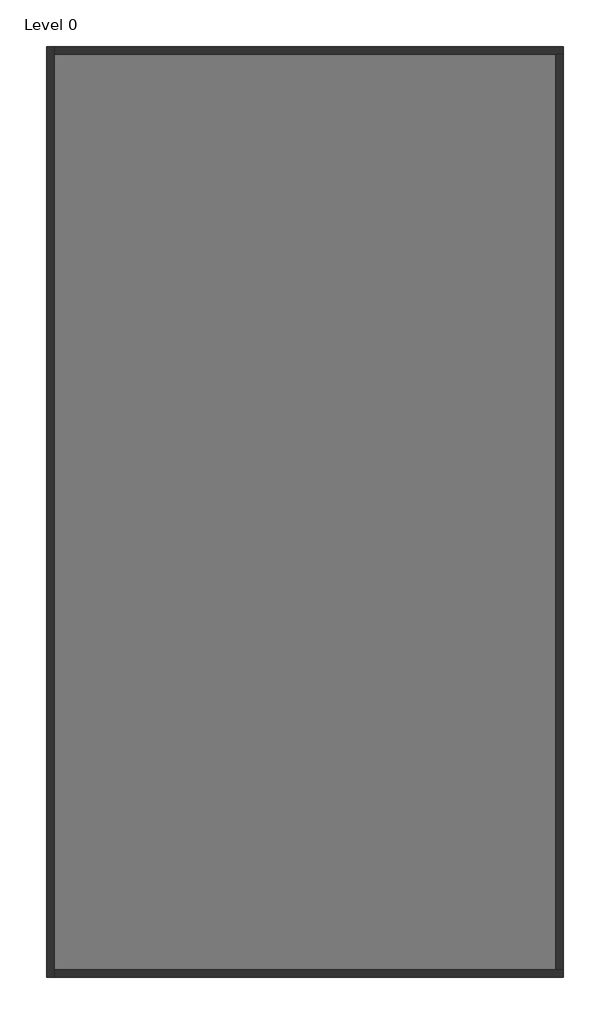
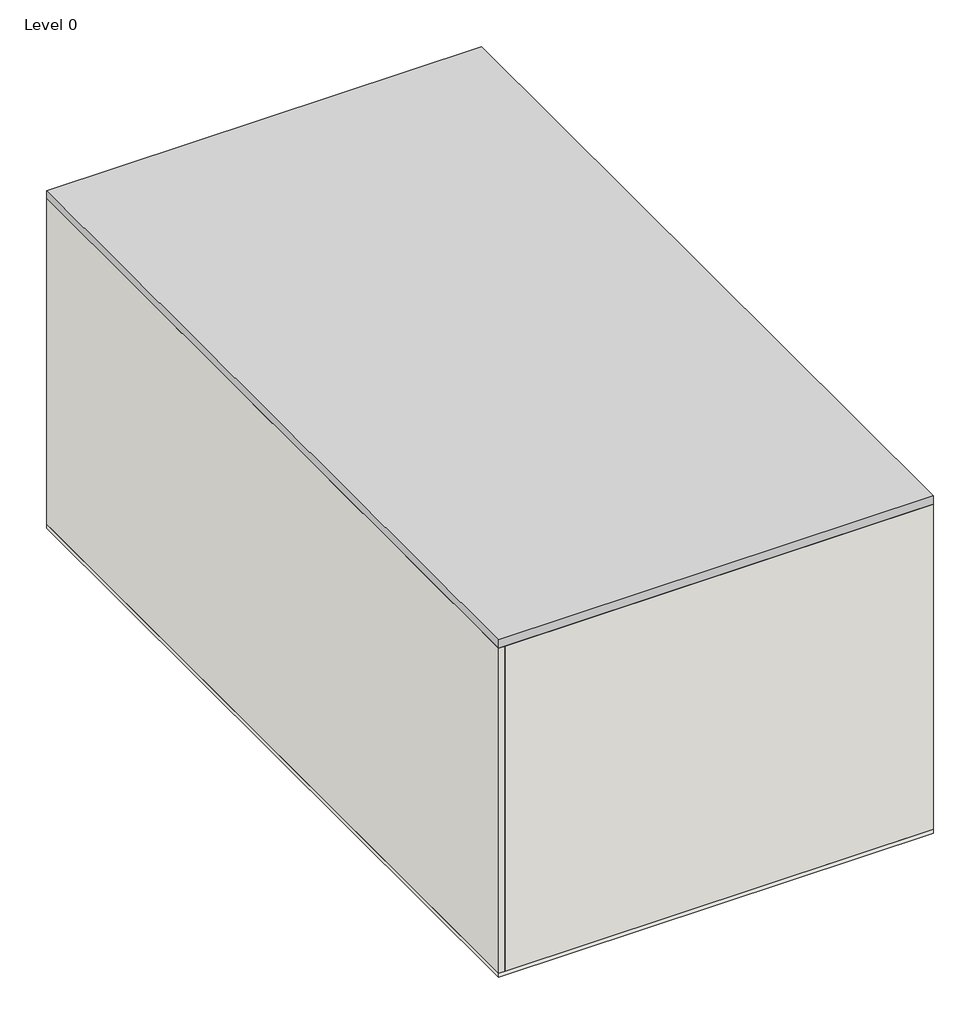
# One storey: 4 walls, 1 proxy, 1 slab.
"""IFC4 building model written with IfcOpenShell, lengths in millimetres."""

from ifc_helpers import new_model, si_unit, frame, origin, origin_with_axes, place, context, project, spatial, polyline, outline, extrude, faceted_brep, element, save

model = new_model("IFC4")

# Units and contexts
model_context = context("Model", 3, world=origin())
ifc_project = project(units=[si_unit("LENGTHUNIT", "METRE", prefix="MILLI")], contexts=[model_context])

# Site, building, storey
site = spatial("IfcSite", under=ifc_project)
building = spatial("IfcBuilding", under=site)
storey = spatial("IfcBuildingStorey", under=building, Name="Level 0", Elevation=100.0)

# Proxy
placement = place(None, origin())
element("IfcBuildingElementProxy", 1, Name="LowUrbanDensityBuilding : LowUrbanDensityBuilding", ObjectType="LowUrbanDensityBuilding : LowUrbanDensityBuilding", at=placement, inside=storey, context=model_context, shape_type="SweptSolid", body=[
    extrude(outline(polyline([(7325.2659446, 3676.2074539), (7325.2659446, -14323.7925461), (-2674.7340554, -14323.7925461), (-2674.7340554, 3676.2074539), (7325.2659446, 3676.2074539)])), origin_with_axes(), (0.0, 0.0, 1.0), 8200.0),
])

# Slab
element("IfcSlab", 2, ObjectType="Floor-Concrete_100Con", at=placement, inside=storey, context=model_context, shape_type="SweptSolid", body=[
    extrude(outline(polyline([(7325.2659446, 3676.2074539), (7325.2659446, -14323.7925461), (-2674.7340554, -14323.7925461), (-2674.7340554, 3676.2074539), (7325.2659446, 3676.2074539)])), origin_with_axes(), (0.0, 0.0, 1.0), 100.0),
])

# Walls
element("IfcWall", 3, ObjectType="Wall-Ext_25Rdr-100Blk-19P", at=placement, inside=storey, context=model_context, shape_type="Brep", body=[
    faceted_brep([(-2674.7340554, 3676.2074539, 100.0), (-2674.7340554, -14323.7925461, 100.0), (-2674.7340554, -14323.7925461, 8000.0), (-2674.7340554, 3676.2074539, 8000.0), (-2530.4340554, 3676.2074539, 100.0), (-2530.4340554, 3676.2074539, 8000.0), (-2530.4340554, 3531.9074539, 8000.0), (-2530.4340554, -14179.4925461, 8000.0), (-2530.4340554, -14323.7925461, 8000.0), (-2530.4340554, -14323.7925461, 100.0), (-2530.4340554, -14179.4925461, 100.0), (-2530.4340554, 3531.9074539, 100.0)], [[[0, 1, 2, 3]], [[4, 5, 6, 7, 8, 9, 10, 11]], [[1, 0, 4, 11, 10, 9]], [[3, 2, 8, 7, 6, 5]], [[2, 1, 9, 8]], [[0, 3, 5, 4]]]),
])
element("IfcWall", 4, ObjectType="Wall-Ext_25Rdr-100Blk-19P", at=placement, inside=storey, context=model_context, shape_type="Brep", body=[
    faceted_brep([(-2530.4340554, -14323.7925461, 100.0), (7325.2659446, -14323.7925461, 100.0), (7325.2659446, -14323.7925461, 8000.0), (-2530.4340554, -14323.7925461, 8000.0), (-2530.4340554, -14179.4925461, 100.0), (-2530.4340554, -14179.4925461, 8000.0), (7180.9659446, -14179.4925461, 8000.0), (7325.2659446, -14179.4925461, 8000.0), (7325.2659446, -14179.4925461, 100.0), (7180.9659446, -14179.4925461, 100.0)], [[[0, 1, 2, 3]], [[4, 5, 6, 7, 8, 9]], [[1, 0, 4, 9, 8]], [[3, 2, 7, 6, 5]], [[0, 3, 5, 4]], [[2, 1, 8, 7]]]),
])
element("IfcWall", 5, ObjectType="Wall-Ext_25Rdr-100Blk-19P", at=placement, inside=storey, context=model_context, shape_type="Brep", body=[
    faceted_brep([(7325.2659446, 3676.2074539, 100.0), (-2530.4340554, 3676.2074539, 100.0), (-2530.4340554, 3676.2074539, 8000.0), (7325.2659446, 3676.2074539, 8000.0), (7325.2659446, 3531.9074539, 100.0), (7325.2659446, 3531.9074539, 8000.0), (7180.9659446, 3531.9074539, 8000.0), (-2530.4340554, 3531.9074539, 8000.0), (-2530.4340554, 3531.9074539, 100.0), (7180.9659446, 3531.9074539, 100.0)], [[[0, 1, 2, 3]], [[4, 5, 6, 7, 8, 9]], [[1, 0, 4, 9, 8]], [[3, 2, 7, 6, 5]], [[2, 1, 8, 7]], [[0, 3, 5, 4]]]),
])
element("IfcWall", 6, ObjectType="Wall-Ext_25Rdr-100Blk-19P", at=placement, inside=storey, context=model_context, shape_type="SweptSolid", body=[
    extrude(outline(polyline([(7325.2659446, 3531.9074539), (7325.2659446, -14179.4925461), (7180.9659446, -14179.4925461), (7180.9659446, 3531.9074539), (7325.2659446, 3531.9074539)])), frame((0.0, 0.0, 100.0), z_axis=(0.0, 0.0, 1.0), x_axis=(1.0, 0.0, 0.0)), (0.0, 0.0, 1.0), 7900.0),
])

save(model, "model.ifc")

# Revit data of these elements
# Project information
#   Project Issue Date = "Issue Date"
#   Project Status = "Project Status"
#   Client Name = "Owner"
#   Project Address = "Enter address here"
#   Project Name = "Project Name"
#   Project Number = "Project Number"
# Type "Floor-Concrete_100Con"
#   Keynote = "E60/130"
#   Function = 0
#   Layers, outside or top first: 100 mm "Concrete" (function 1)
# Type "Wall-Ext_25Rdr-100Blk-19P"
#   Keynote = "F10"
#   Layers, outside or top first: 25.3 mm "Render, Beige, Smooth" (function 5); 100 mm "Concrete Masonry Units _Low Density" (function 1); 19 mm "Plaster" (function 5)
# Element 1 (IfcBuildingElementProxy, "LowUrbanDensityBuilding : LowUrbanDensityBuilding")
#   Phase Created = New Construction
#   Materials on its faces: "Default Form"
# Element 2 (IfcSlab, "Floor-Concrete_100Con")
#   Height Offset From Level = 0 mm
#   Phase Created = New Construction
#   Materials on its faces: "Concrete"
# Element 3 (IfcWall, "Wall-Ext_25Rdr-100Blk-19P")
#   Top Offset = 0 mm
#   Base Offset = 0 mm
#   wall height = 7900 mm
#   Phase Created = New Construction
#   Base Constraint = Level 0
#   Top Constraint = Level 2
#   Materials on its faces: "Render, Beige, Smooth", "Default Wall", "Plaster"
# Elements 4, 5, 6 (IfcWall, "Wall-Ext_25Rdr-100Blk-19P")
#   Top Offset = 0 mm
#   Base Offset = 0 mm
#   wall height = 7900 mm
#   Phase Created = New Construction
#   Base Constraint = Level 0
#   Top Constraint = Level 2
#   Materials on its faces: "Default Wall", "Render, Beige, Smooth", "Plaster"
# Materials
#   "Concrete": class "Concrete", colour RGB 120 120 120, transparency 0, Description = "Portland Cement Concrete", Cost = 0
#   "Render, Beige, Smooth": class "Generic", colour RGB 213 198 180, transparency 0, Description = "physical material", Cost = 0
#   "Concrete Masonry Units _Low Density": class "Masonry", colour RGB 181 181 181, transparency 0, Description = "Concrete masonry units", Cost = 0
#   "Plaster": class "Generic", colour RGB 249 249 249, transparency 0, Description = "Plaster", Cost = 0
#   "Default Form": class "Generic", colour RGB 185 189 196, transparency 0.5, Cost = 0
#   "Default Wall": class "Miscellaneous", colour RGB 128 128 128, transparency 0, Comments = "Rendering appearance not upgraded Rendering appearance not upgraded ", Cost = 0
